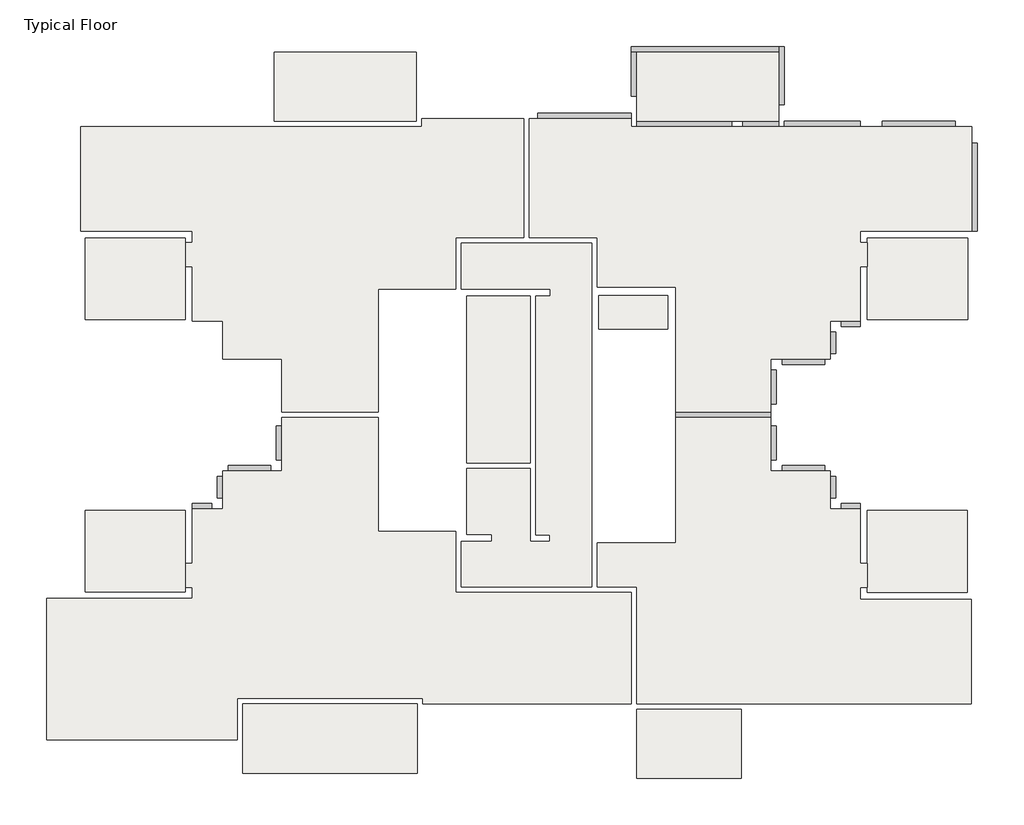
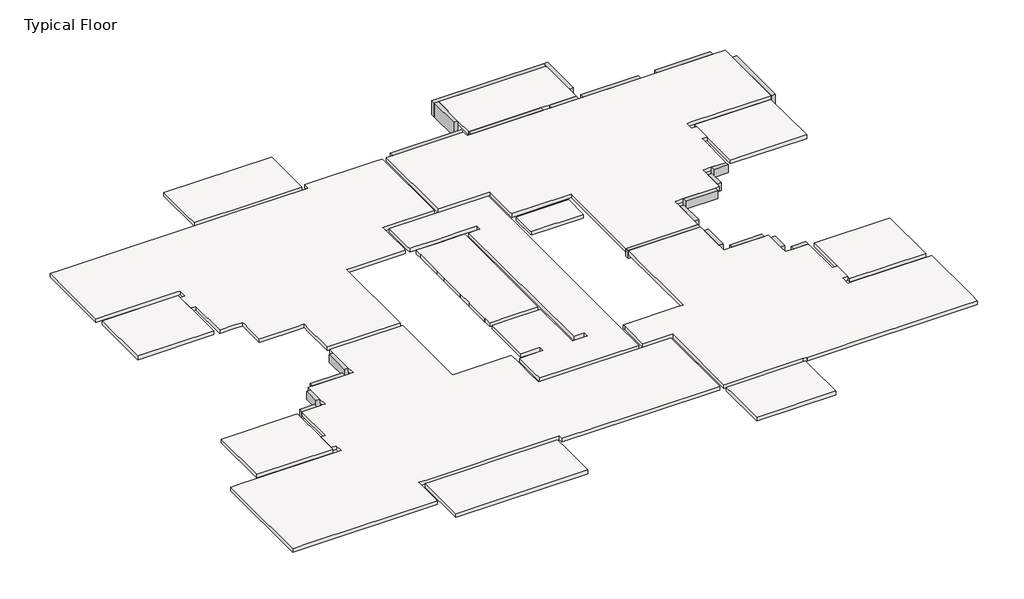
# One storey: 22 beams, 15 slabs.
# Revit data of these elements (continued)
# Element 2 (IfcBeam, "Concrete Rectengular Beam : 20/40") (continued)
#   Phase Created = New Construction
#   Materials on its faces: "Concrete"
# Element 3 (IfcBeam, "Concrete Rectengular Beam : 20/40")
#   Comments = ""
#   Mark = "B8"
#   SOFiSTiK_AMG_Comments = ""
#   SOFiSTiK_AMG_Scheduled = yes
#   SOFiSTiK_AMG_Adjusted = yes
#   Structural Material = Concrete
#   Phase Created = New Construction
#   Materials on its faces: "Concrete"
# Element 4 (IfcBeam, "Concrete Rectengular Beam : 20/40")
#   Comments = ""
#   Mark = "B9"
#   SOFiSTiK_AMG_Comments = ""
#   SOFiSTiK_AMG_Scheduled = yes
#   SOFiSTiK_AMG_Adjusted = yes
#   Structural Material = Concrete
#   Phase Created = New Construction
#   Materials on its faces: "Concrete"
# Element 5 (IfcBeam, "Concrete Rectengular Beam : 20/40")
#   Comments = ""
#   Mark = "B10"
#   SOFiSTiK_AMG_Comments = ""
#   SOFiSTiK_AMG_Scheduled = yes
#   SOFiSTiK_AMG_Adjusted = yes
#   Structural Material = Concrete
#   Phase Created = New Construction
#   Materials on its faces: "Concrete"
# Element 6 (IfcBeam, "Concrete Rectengular Beam : 20/40")
#   Comments = ""
#   Mark = "B11"
#   SOFiSTiK_AMG_Comments = ""
#   SOFiSTiK_AMG_Scheduled = yes
#   SOFiSTiK_AMG_Adjusted = yes
#   Structural Material = Concrete
#   Phase Created = New Construction
#   Materials on its faces: "Concrete"
# Element 7 (IfcBeam, "Concrete Rectengular Beam : 20/40")
#   Comments = ""
#   Mark = "B12"
#   SOFiSTiK_AMG_Comments = ""
#   SOFiSTiK_AMG_Scheduled = yes
#   SOFiSTiK_AMG_Adjusted = yes
#   Structural Material = Concrete
#   Phase Created = New Construction
#   Materials on its faces: "Concrete"
# Element 8 (IfcBeam, "Concrete Rectengular Beam : 20/40")
#   Comments = ""
#   Mark = "B13"
#   SOFiSTiK_AMG_Comments = ""
#   SOFiSTiK_AMG_Scheduled = yes
#   SOFiSTiK_AMG_Adjusted = yes
#   Structural Material = Concrete
#   Phase Created = New Construction
#   Materials on its faces: "Concrete"
# Element 9 (IfcBeam, "Concrete Rectengular Beam : 20/40")
#   Comments = ""
#   Mark = "B14"
#   SOFiSTiK_AMG_Comments = ""
#   SOFiSTiK_AMG_Scheduled = yes
#   SOFiSTiK_AMG_Adjusted = yes
#   Structural Material = Concrete
#   Phase Created = New Construction
#   Materials on its faces: "Concrete"
# Element 10 (IfcBeam, "Concrete Rectengular Beam : 20/40")
#   Comments = ""
#   Mark = "B15"
#   SOFiSTiK_AMG_Comments = ""
#   SOFiSTiK_AMG_Scheduled = yes
#   SOFiSTiK_AMG_Adjusted = yes
#   Structural Material = Concrete
#   Phase Created = New Construction
#   Materials on its faces: "Concrete"
# Element 11 (IfcBeam, "Concrete Rectengular Beam : 20/40")
#   Comments = ""
#   Mark = "B16"
#   SOFiSTiK_AMG_Comments = ""
#   SOFiSTiK_AMG_Scheduled = yes
#   SOFiSTiK_AMG_Adjusted = yes
#   Structural Material = Concrete
#   Phase Created = New Construction
#   Materials on its faces: "Concrete"
# Element 12 (IfcBeam, "Concrete Rectengular Beam : 20/40")
#   Comments = ""
#   Mark = "B17"
#   SOFiSTiK_AMG_Comments = ""
#   SOFiSTiK_AMG_Scheduled = yes
#   SOFiSTiK_AMG_Adjusted = yes
#   Structural Material = Concrete
#   Phase Created = New Construction
#   Materials on its faces: "Concrete"
# Element 13 (IfcBeam, "Concrete Rectengular Beam : 20/40")
#   Comments = ""
#   Mark = "B18"
#   SOFiSTiK_AMG_Comments = ""
#   SOFiSTiK_AMG_Scheduled = yes
#   SOFiSTiK_AMG_Adjusted = yes
#   Structural Material = Concrete
#   Phase Created = New Construction
#   Materials on its faces: "Concrete"
# Element 14 (IfcBeam, "Concrete Rectengular Beam : 20/50")
#   Comments = ""
#   Mark = "B30"
#   SOFiSTiK_AMG_Comments = ""
#   SOFiSTiK_AMG_Scheduled = yes
#   SOFiSTiK_AMG_Adjusted = yes
#   Structural Material = Concrete
#   Phase Created = New Construction
#   Materials on its faces: "Concrete"
# Element 15 (IfcBeam, "Concrete Rectengular Beam : 20/50")
#   Comments = ""
#   Mark = "B31"
#   SOFiSTiK_AMG_Comments = ""
#   SOFiSTiK_AMG_Scheduled = yes
#   SOFiSTiK_AMG_Adjusted = yes
#   Structural Material = Concrete
#   Phase Created = New Construction
#   Materials on its faces: "Concrete"
# Element 16 (IfcBeam, "Concrete Rectengular Beam : 20/50")
#   Comments = ""
#   Mark = "B32"
#   SOFiSTiK_AMG_Comments = ""
#   SOFiSTiK_AMG_Scheduled = yes
#   SOFiSTiK_AMG_Adjusted = yes
#   Structural Material = Concrete
#   Phase Created = New Construction
#   Materials on its faces: "Concrete"
# Element 17 (IfcBeam, "Concrete Rectengular Beam : 20/50")
#   Comments = ""
#   Mark = "B33"
#   SOFiSTiK_AMG_Comments = ""
#   SOFiSTiK_AMG_Scheduled = yes
#   SOFiSTiK_AMG_Adjusted = yes
#   Structural Material = Concrete
#   Phase Created = New Construction
#   Materials on its faces: "Concrete"
# Element 18 (IfcBeam, "Concrete Rectengular Beam : 20/50")
#   Comments = ""
#   Mark = "B34"
#   SOFiSTiK_AMG_Comments = ""
#   SOFiSTiK_AMG_Scheduled = yes
#   SOFiSTiK_AMG_Adjusted = yes
#   Structural Material = Concrete
#   Phase Created = New Construction
#   Materials on its faces: "Concrete"
# Element 19 (IfcBeam, "Concrete Rectengular Beam : 20/50")
#   Comments = ""
#   Mark = "B35"
#   SOFiSTiK_AMG_Comments = ""
#   SOFiSTiK_AMG_Scheduled = yes
#   SOFiSTiK_AMG_Adjusted = yes
#   Structural Material = Concrete
#   Phase Created = New Construction
#   Materials on its faces: "Concrete"
# Element 20 (IfcBeam, "Concrete Rectengular Beam : 20/70")
#   Comments = ""
#   Mark = "B52"
#   SOFiSTiK_AMG_Comments = ""
#   SOFiSTiK_AMG_Scheduled = yes
#   SOFiSTiK_AMG_Adjusted = yes
#   Structural Material = Concrete
#   Phase Created = New Construction
#   Materials on its faces: "Concrete"
# Element 21 (IfcBeam, "Concrete Rectengular Beam : 20/70")
#   Comments = ""
#   Mark = "B53"
#   SOFiSTiK_AMG_Comments = ""
#   SOFiSTiK_AMG_Scheduled = yes
#   SOFiSTiK_AMG_Adjusted = yes
#   Structural Material = Concrete
#   Phase Created = New Construction
#   Materials on its faces: "Concrete"
# Element 22 (IfcBeam, "Concrete Rectengular Beam : 20/70")
#   Comments = ""
#   Mark = "B54"
#   SOFiSTiK_AMG_Comments = ""
#   SOFiSTiK_AMG_Scheduled = yes
#   SOFiSTiK_AMG_Adjusted = yes
#   Structural Material = Concrete
#   Phase Created = New Construction
#   Materials on its faces: "Concrete"
# Element 23 (IfcSlab, "18")
#   Mark = "S1"
#   SOFiSTiK_AMG_Comments = ""
#   Height Offset From Level = 0 cm
#   built-in parameter 1001954 = 1
#   SOFiSTiK_AMG_Scheduled = yes
#   SOFiSTiK_AMG_Adjusted = yes
#   Phase Created = New Construction
#   Materials on its faces: "Concrete"
# Element 24 (IfcSlab, "18")
#   Mark = "S2"
#   SOFiSTiK_AMG_Comments = ""
#   built-in parameter 1001955 = -1.5708 (stored number, unit not read)
#   Height Offset From Level = 0 cm
#   built-in parameter 1001954 = 1
#   SOFiSTiK_AMG_Scheduled = yes
#   SOFiSTiK_AMG_Adjusted = yes
#   Phase Created = New Construction
#   Materials on its faces: "Concrete"
# Element 25 (IfcSlab, "18")
#   Mark = "S3"
#   SOFiSTiK_AMG_Comments = ""
#   Height Offset From Level = 0 cm
#   built-in parameter 1001954 = 1
#   SOFiSTiK_AMG_Scheduled = yes
#   SOFiSTiK_AMG_Adjusted = yes
#   Phase Created = New Construction
#   Materials on its faces: "Concrete"
# Element 26 (IfcSlab, "18")
#   Mark = "S4"
#   SOFiSTiK_AMG_Comments = ""
#   built-in parameter 1001955 = 3.14159 (stored number, unit not read)
#   Height Offset From Level = 0 cm
#   built-in parameter 1001954 = 1
#   SOFiSTiK_AMG_Scheduled = yes
#   SOFiSTiK_AMG_Adjusted = yes
#   Phase Created = New Construction
#   Materials on its faces: "Concrete"
# Element 27 (IfcSlab, "18")
#   Mark = "S5"
#   SOFiSTiK_AMG_Comments = ""
#   built-in parameter 1001955 = -1.5708 (stored number, unit not read)
#   Height Offset From Level = 0 cm
#   built-in parameter 1001954 = 1
#   SOFiSTiK_AMG_Scheduled = yes
#   SOFiSTiK_AMG_Adjusted = yes
#   Phase Created = New Construction
#   Materials on its faces: "Concrete"
# Element 28 (IfcSlab, "18")
#   Mark = "S6"
#   SOFiSTiK_AMG_Comments = ""
#   built-in parameter 1001955 = 3.14159 (stored number, unit not read)
#   Height Offset From Level = 0 cm
#   built-in parameter 1001954 = 1
#   SOFiSTiK_AMG_Scheduled = yes
#   SOFiSTiK_AMG_Adjusted = yes
#   Phase Created = New Construction
#   Materials on its faces: "Concrete"
# Element 29 (IfcSlab, "18")
#   Mark = "S7"
#   SOFiSTiK_AMG_Comments = ""
#   Height Offset From Level = 0 cm
#   built-in parameter 1001954 = 1
#   SOFiSTiK_AMG_Scheduled = yes
#   SOFiSTiK_AMG_Adjusted = yes
#   Phase Created = New Construction
#   Materials on its faces: "Concrete"
# Element 30 (IfcSlab, "18")
#   Mark = "S8"
#   SOFiSTiK_AMG_Comments = ""
#   built-in parameter 1001955 = 3.14159 (stored number, unit not read)
#   Height Offset From Level = 0 cm
#   built-in parameter 1001954 = 1
#   SOFiSTiK_AMG_Scheduled = yes
#   SOFiSTiK_AMG_Adjusted = yes
#   Phase Created = New Construction
#   Materials on its faces: "Concrete"
# Element 31 (IfcSlab, "18")
#   Mark = "S9"
#   SOFiSTiK_AMG_Comments = ""
#   built-in parameter 1001955 = 1.5708 (stored number, unit not read)
#   Height Offset From Level = 0 cm
#   built-in parameter 1001954 = 1
#   SOFiSTiK_AMG_Scheduled = yes
#   SOFiSTiK_AMG_Adjusted = yes
#   Phase Created = New Construction
#   Materials on its faces: "Concrete"
# Element 32 (IfcSlab, "18")
#   Mark = "S10"
#   SOFiSTiK_AMG_Comments = ""
#   Height Offset From Level = 0 cm
#   built-in parameter 1001954 = 1
#   SOFiSTiK_AMG_Scheduled = yes
#   SOFiSTiK_AMG_Adjusted = yes
#   Phase Created = New Construction
#   Materials on its faces: "Concrete"
# Element 33 (IfcSlab, "18")
#   Mark = "S11"
#   SOFiSTiK_AMG_Comments = ""
#   Height Offset From Level = 0 cm
#   built-in parameter 1001954 = 1
#   SOFiSTiK_AMG_Scheduled = yes
#   SOFiSTiK_AMG_Adjusted = yes
#   Phase Created = New Construction
#   Materials on its faces: "Concrete"
# Element 34 (IfcSlab, "18")
#   Mark = "S12"
#   SOFiSTiK_AMG_Comments = ""
#   Height Offset From Level = 0 cm
#   built-in parameter 1001954 = 1
#   SOFiSTiK_AMG_Scheduled = yes
#   SOFiSTiK_AMG_Adjusted = yes
#   Phase Created = New Construction
#   Materials on its faces: "Concrete"
# Element 35 (IfcSlab, "18")
#   Mark = "S13"
#   SOFiSTiK_AMG_Comments = ""
#   Height Offset From Level = 0 cm
#   built-in parameter 1001954 = 1
#   SOFiSTiK_AMG_Scheduled = yes
#   SOFiSTiK_AMG_Adjusted = yes
#   Phase Created = New Construction
#   Materials on its faces: "Concrete"
# Element 36 (IfcSlab, "18")
#   Mark = "S14"
#   SOFiSTiK_AMG_Comments = ""
#   Height Offset From Level = 0 cm
#   built-in parameter 1001954 = 1
#   SOFiSTiK_AMG_Scheduled = yes
#   SOFiSTiK_AMG_Adjusted = yes
#   Phase Created = New Construction
#   Materials on its faces: "Concrete"
# Element 37 (IfcSlab, "18")
#   Mark = "S15"
#   SOFiSTiK_AMG_Comments = ""
#   Height Offset From Level = 0 cm
#   built-in parameter 1001954 = 1
#   SOFiSTiK_AMG_Scheduled = yes
#   SOFiSTiK_AMG_Adjusted = yes
#   Phase Created = New Construction
#   Materials on its faces: "Concrete"
# Materials
#   "Concrete": class "Concrete", colour RGB 192 192 192, transparency 0, Keynote = "01000", Description = "Cast-in-place concrete", Cost = 0
